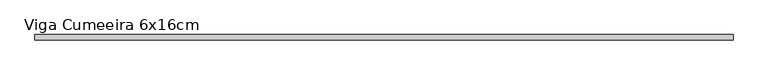
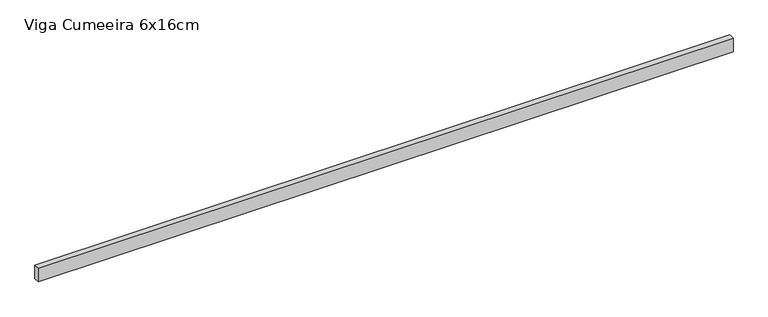
"""IFC4 building model written with IfcOpenShell, lengths in millimetres: beam geometry, Madeira de lei : Viga Cumeeira 6x16cm."""

import ifcopenshell
import ifcopenshell.guid

model = None  # the IFC model being written
_history = None  # IfcOwnerHistory: only IFC2X3 demands one
_inside = {}  # id of a spatial element -> (the spatial element, [elements in it])
_under = {}  # id of a project, library or spatial element -> (it, [spatial elements below it])
_declared = {}  # id of a project -> (the project, [libraries it declares])
_typed = {}  # id of a type object -> (the type object, [elements of that type])
_made_of = {}  # id of a material, layer set ... -> (it, [elements and type objects made of it])


def new_model(schema):
    """Start an empty IFC model of exactly this schema.

    Asked for "IFC4X3", IfcOpenShell would pick the latest addendum, in which some entities
    have other attributes; the version numbers below select the first issue.
    IFC2X3 requires an IfcOwnerHistory on every rooted entity: one is made here for all.
    """
    global model, _history
    if schema == "IFC4X3":
        model = ifcopenshell.file(schema_version=(4, 3, 0, 0))
    else:
        model = ifcopenshell.file(schema=schema)
    _inside.clear()
    _under.clear()
    _declared.clear()
    _typed.clear()
    _made_of.clear()
    _history = None
    if model.schema == "IFC2X3":
        org = make("IfcOrganization", Name="unknown")
        user = make(
            "IfcPersonAndOrganization",
            ThePerson=make("IfcPerson", FamilyName="unknown"),
            TheOrganization=org,
        )
        app = make(
            "IfcApplication",
            ApplicationDeveloper=org,
            Version="unknown",
            ApplicationFullName="unknown",
            ApplicationIdentifier="unknown",
        )
        _history = make(
            "IfcOwnerHistory",
            OwningUser=user,
            OwningApplication=app,
            ChangeAction="ADDED",
            CreationDate=0,
        )
    return model


def make(cls, **values):
    """One entity of the class cls with the attributes given. An attribute that is None is left unset."""
    return model.create_entity(
        cls, **{name: value for name, value in values.items() if value is not None}
    )


def rooted(cls, **values):
    """An entity with a GlobalId (a new one), such as an element, a storey or a relation."""
    return make(cls, GlobalId=ifcopenshell.guid.new(), OwnerHistory=_history, **values)


def si_unit(unit_type, name, prefix=None):
    """IfcSIUnit, for example si_unit("LENGTHUNIT", "METRE", prefix="MILLI")."""
    return make("IfcSIUnit", UnitType=unit_type, Prefix=prefix, Name=name)


def assignment(units):
    """IfcUnitAssignment: the units of a project."""
    return None if units is None else make("IfcUnitAssignment", Units=units)


def point(xyz):
    """IfcCartesianPoint."""
    return None if xyz is None else make("IfcCartesianPoint", Coordinates=xyz)


def direction(xyz):
    """IfcDirection."""
    return None if xyz is None else make("IfcDirection", DirectionRatios=xyz)


def frame(location, z_axis=None, x_axis=None):
    """IfcAxis2Placement3D, a coordinate frame: its origin and axes. An axis left out is left unset."""
    return make(
        "IfcAxis2Placement3D",
        Location=point(location),
        Axis=direction(z_axis),
        RefDirection=direction(x_axis),
    )


def origin():
    """The frame at (0, 0, 0) with its axes left unset."""
    return frame((0.0, 0.0, 0.0))


def place(relative_to, where):
    """IfcLocalPlacement: puts the frame where relative to a parent placement (None: the world)."""
    return make(
        "IfcLocalPlacement", PlacementRelTo=relative_to, RelativePlacement=where
    )


def context(
    kind, dimensions, precision=None, world=None, true_north=None, identifier=None
):
    """IfcGeometricRepresentationContext, for example the 3D "Model" context."""
    return make(
        "IfcGeometricRepresentationContext",
        ContextIdentifier=identifier,
        ContextType=kind,
        CoordinateSpaceDimension=dimensions,
        Precision=precision,
        WorldCoordinateSystem=world,
        TrueNorth=true_north,
    )


def project(units=None, contexts=None):
    """IfcProject with its units and contexts."""
    return rooted(
        "IfcProject",
        Name="project",
        RepresentationContexts=contexts,
        UnitsInContext=assignment(units),
    )


def spatial(cls, under=None, at=None, **own):
    """A site, building, storey or space (cls), placed at a placement, below another one or the project."""
    s = rooted(cls, ObjectPlacement=at, **own)
    if under is not None:
        _under.setdefault(under.id(), (under, []))[1].append(s)
    return s


def polyline(points):
    """IfcPolyline through the points."""
    return make("IfcPolyline", Points=[point(p) for p in points])


def outline(outer, holes=None, kind="AREA"):
    """IfcArbitraryClosedProfileDef: a profile drawn as a closed curve; with holes, ...WithVoids."""
    if holes is None:
        return make("IfcArbitraryClosedProfileDef", ProfileType=kind, OuterCurve=outer)
    return make(
        "IfcArbitraryProfileDefWithVoids",
        ProfileType=kind,
        OuterCurve=outer,
        InnerCurves=holes,
    )


def extrude(swept, where, along, depth):
    """IfcExtrudedAreaSolid: the profile swept, set in the frame where, extruded along a direction by depth."""
    return make(
        "IfcExtrudedAreaSolid",
        SweptArea=swept,
        Position=where,
        ExtrudedDirection=direction(along),
        Depth=depth,
    )


def shape(context_of_items, identifier, shape_type, items):
    """IfcShapeRepresentation: the items that make up one representation, for example the "Body"."""
    return make(
        "IfcShapeRepresentation",
        ContextOfItems=context_of_items,
        RepresentationIdentifier=identifier,
        RepresentationType=shape_type,
        Items=items,
    )


def source(mapping_origin, context_of_items, identifier, shape_type, items):
    """IfcRepresentationMap: a shape defined once, which mapped items show again and again."""
    return make(
        "IfcRepresentationMap",
        MappingOrigin=mapping_origin,
        MappedRepresentation=shape(context_of_items, identifier, shape_type, items),
    )


def transform(
    local_origin,
    x_axis=None,
    y_axis=None,
    z_axis=None,
    scale=None,
    scale2=None,
    scale3=None,
    uniform=True,
):
    """IfcCartesianTransformationOperator3D, or its non-uniform kind. x_axis, y_axis, z_axis: its Axis1, 2, 3."""
    if uniform:
        return make(
            "IfcCartesianTransformationOperator3D",
            Axis1=direction(x_axis),
            Axis2=direction(y_axis),
            LocalOrigin=point(local_origin),
            Scale=scale,
            Axis3=direction(z_axis),
        )
    return make(
        "IfcCartesianTransformationOperator3DnonUniform",
        Axis1=direction(x_axis),
        Axis2=direction(y_axis),
        LocalOrigin=point(local_origin),
        Scale=scale,
        Axis3=direction(z_axis),
        Scale2=scale2,
        Scale3=scale3,
    )


def mapped(mapping_source, mapping_target):
    """IfcMappedItem: shows the shape of a source again, moved by a transform."""
    return make(
        "IfcMappedItem", MappingSource=mapping_source, MappingTarget=mapping_target
    )


def made_of(thing, what):
    """Note that an element or type object is made of a material, layer set ...; save() writes the relation."""
    if what is not None:
        _made_of.setdefault(what.id(), (what, []))[1].append(thing)
    return thing


def element(
    cls,
    number,
    at=None,
    inside=None,
    cuts=None,
    type_object=None,
    material=None,
    context=None,
    identifier="Body",
    shape_type=None,
    held_by="IfcProductDefinitionShape",
    body=None,
    shapes=None,
    **own,
):
    """One element of the class cls, such as IfcWall. Its Tag is "e" and its number.

    at: its placement. inside: the storey or other place that contains it. cuts: it is an
    opening in that element (IfcRelVoidsElement). A single representation is given by context,
    identifier, shape_type and body (its items); several are given by shapes. held_by: the class
    of the entity that holds the representations. save() writes the other relations.
    """
    e = rooted(cls, Tag="e%d" % number, ObjectPlacement=at, **own)
    if body is not None:
        shapes = [shape(context, identifier, shape_type, body)]
    if shapes is not None:
        e.Representation = make(held_by, Representations=shapes)
    if inside is not None:
        _inside.setdefault(inside.id(), (inside, []))[1].append(e)
    if cuts is not None:
        rooted(
            "IfcRelVoidsElement", RelatingBuildingElement=cuts, RelatedOpeningElement=e
        )
    if type_object is not None:
        _typed.setdefault(type_object.id(), (type_object, []))[1].append(e)
    return made_of(e, material)


def aggregate(whole, parts):
    """IfcRelAggregates: a whole, such as a stair, and the parts it consists of."""
    return rooted("IfcRelAggregates", RelatingObject=whole, RelatedObjects=parts)


def save(model, path):
    """Write the relations noted so far, then the file.

    IfcRelAggregates (storeys below a building ...), IfcRelContainedInSpatialStructure (elements
    in a storey), IfcRelDefinesByType, IfcRelAssociatesMaterial and IfcRelDeclares: one each for
    every whole, place, type object, material and project.
    """
    for whole, parts in _under.values():
        aggregate(whole, parts)
    for where, things in _inside.values():
        rooted(
            "IfcRelContainedInSpatialStructure",
            RelatedElements=things,
            RelatingStructure=where,
        )
    for kind, things in _typed.values():
        rooted("IfcRelDefinesByType", RelatedObjects=things, RelatingType=kind)
    for what, things in _made_of.values():
        rooted("IfcRelAssociatesMaterial", RelatedObjects=things, RelatingMaterial=what)
    for by, libraries in _declared.values():
        rooted("IfcRelDeclares", RelatingContext=by, RelatedDefinitions=libraries)
    model.write(path)


def viga_cumeeira_6x16cm_8fcfcc43(model_context):
    return source(origin(), model_context, "Body", "SweptSolid", [
        extrude(outline(polyline([(3822.5, 30.0), (3822.5, -30.0), (-3822.5, -30.0), (-3822.5, 30.0), (3822.5, 30.0)])), frame((0.0, 0.0, -80.0), z_axis=(0.0, 0.0, 1.0), x_axis=(1.0, 0.0, 0.0)), (0.0, 0.0, 1.0), 160.0),
    ])


if __name__ == "__main__":
    model = new_model("IFC4")
    model_context = context("Model", 3, world=origin())
    ifc_project = project(units=[si_unit("LENGTHUNIT", "METRE", prefix="MILLI")], contexts=[model_context])
    site = spatial("IfcSite", under=ifc_project)
    building = spatial("IfcBuilding", under=site)
    placement = place(None, origin())
    viga_cumeeira_6x16cm_shape = viga_cumeeira_6x16cm_8fcfcc43(model_context)
    element("IfcBeam", 1, ObjectType="Madeira de lei : Viga Cumeeira 6x16cm", at=placement, inside=building, context=model_context, shape_type="MappedRepresentation", body=[
        mapped(viga_cumeeira_6x16cm_shape, transform((0.0, 0.0, 0.0), x_axis=(1.0, 0.0, 0.0), y_axis=(0.0, 1.0, 0.0), z_axis=(0.0, 0.0, 1.0))),
    ])
    save(model, "model.ifc")

# Revit data of these elements
# Type "Madeira de lei : Viga Cumeeira 6x16cm"
#   A = 0.02 m²
#   Length [instance default] = 1.524 m
#   b = 0.06 m
#   d = 0.16 m
#   Structural Material [instance default] = none
#   Assembly Code = ""
# Element 1 (IfcBeam, "Madeira de lei : Viga Cumeeira 6x16cm")
#   Structural Material = .MADEIRAMENTO
#   Materials on its faces: ".MADEIRAMENTO"
# Materials
#   ".MADEIRAMENTO": class ".CC_MADEIRAS", colour RGB 212 179 113, transparency 0, Cost = 0
